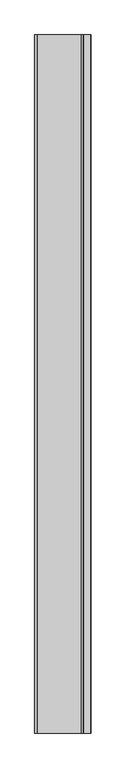
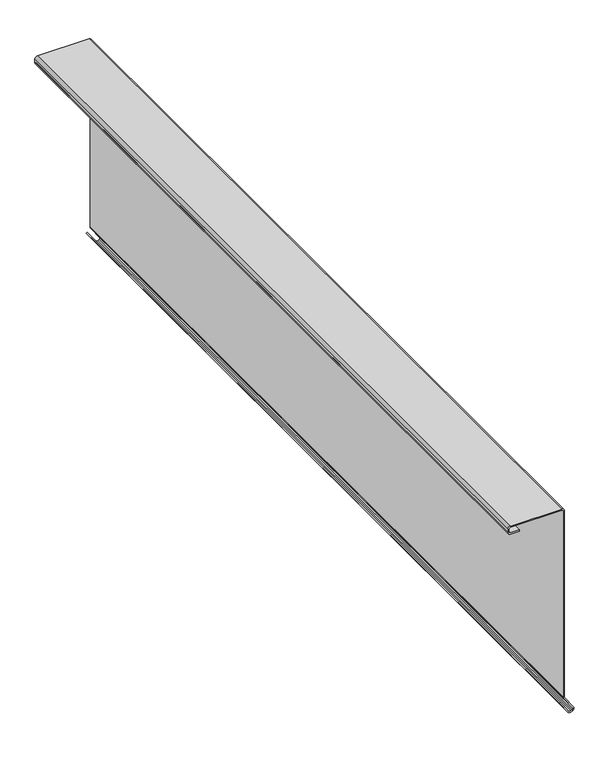
"""IFC4 building model written with IfcOpenShell, lengths in millimetres: proxy geometry, Flashing18:Flashing024:302126 : Flashing18:Flashing024:302126."""

from ifc_helpers import new_model, si_unit, point, frame, frame_2d, origin, place, context, project, spatial, polyline, circle_curve, trimmed, segment, composite_curve, outline, extrude, source, transform, mapped, element, save


def generic_models_c848868d(model_context):
    return source(origin(), model_context, "Body", "SweptSolid", [
        extrude(outline(composite_curve([segment(polyline([(41350.6549147, 10934.2276149), (41320.2092308, 10955.7821514)]), True, "CONTINUOUS"), segment(trimmed(circle_curve(frame_2d((41323.8783762, 10960.9648024)), 6.35), [point((41320.2092308, 10955.7821514))], [point((41318.4012804, 10964.1778884))], False, "CARTESIAN"), True, "CONTINUOUS"), segment(polyline([(41318.4012804, 10964.1778884), (41320.1425067, 10967.1460205)]), True, "CONTINUOUS"), segment(trimmed(circle_curve(frame_2d((41325.6196026, 10963.9329345)), 6.35), [point((41320.1425067, 10967.1460205))], [point((41329.2370767, 10969.1517831))], False, "CARTESIAN"), True, "CONTINUOUS"), segment(polyline([(41329.2370767, 10969.1517831), (41359.2301171, 10948.3619391)]), True, "CONTINUOUS"), segment(trimmed(circle_curve(frame_2d((41362.8475913, 10953.5807877)), 6.35), [point((41359.2301171, 10948.3619391))], [point((41362.8475913, 10947.2307877))], True, "CARTESIAN"), True, "CONTINUOUS"), segment(polyline([(41362.8475913, 10947.2307877), (41842.9189039, 10947.2307877)]), True, "CONTINUOUS"), segment(trimmed(circle_curve(frame_2d((41842.9189039, 10940.8807877)), 6.35), [point((41842.9189039, 10947.2307877))], [point((41849.2689039, 10940.8807877))], False, "CARTESIAN"), True, "CONTINUOUS"), segment(polyline([(41849.2689039, 10940.8807877), (41849.2689039, 10815.1631684)]), True, "CONTINUOUS"), segment(trimmed(circle_curve(frame_2d((41842.9189039, 10815.1631684)), 6.35), [point((41849.2689039, 10815.1631684))], [point((41842.9189039, 10808.8131684))], False, "CARTESIAN"), True, "CONTINUOUS"), segment(polyline([(41842.9189039, 10808.8131684), (41835.0524976, 10808.8131684)]), True, "CONTINUOUS"), segment(trimmed(circle_curve(frame_2d((41835.0524976, 10815.1631684)), 6.35), [point((41835.0524976, 10808.8131684))], [point((41828.7024976, 10815.1631684))], False, "CARTESIAN"), True, "CONTINUOUS"), segment(polyline([(41828.7024976, 10815.1631684), (41828.7024976, 10837.1896333), (41831.7024976, 10837.1896333), (41831.7024976, 10815.1631685)]), True, "CONTINUOUS"), segment(trimmed(circle_curve(frame_2d((41835.0524976, 10815.1631685)), 3.35), [point((41831.7024976, 10815.1631685))], [point((41835.0524976, 10811.8131685))], True, "CARTESIAN"), True, "CONTINUOUS"), segment(polyline([(41835.0524976, 10811.8131685), (41842.9189039, 10811.8131685)]), True, "CONTINUOUS"), segment(trimmed(circle_curve(frame_2d((41842.9189039, 10815.1631685)), 3.35), [point((41842.9189039, 10811.8131685))], [point((41846.2689039, 10815.1631685))], True, "CARTESIAN"), True, "CONTINUOUS"), segment(polyline([(41846.2689039, 10815.1631685), (41846.2689039, 10940.8807877)]), True, "CONTINUOUS"), segment(trimmed(circle_curve(frame_2d((41842.9189039, 10940.8807877)), 3.35), [point((41846.2689039, 10940.8807877))], [point((41842.9189039, 10944.2307877))], True, "CARTESIAN"), True, "CONTINUOUS"), segment(polyline([(41842.9189039, 10944.2307877), (41362.8475913, 10944.2307877)]), True, "CONTINUOUS"), segment(trimmed(circle_curve(frame_2d((41362.8475913, 10953.5807877)), 9.35), [point((41362.8475913, 10944.2307877))], [point((41357.5210742, 10945.8963413))], False, "CARTESIAN"), True, "CONTINUOUS"), segment(polyline([(41357.5210742, 10945.8963413), (41327.5280338, 10966.6861854)]), True, "CONTINUOUS"), segment(trimmed(circle_curve(frame_2d((41325.6196026, 10963.9329345)), 3.35), [point((41327.5280338, 10966.6861854))], [point((41322.730111, 10965.6280271))], True, "CARTESIAN"), True, "CONTINUOUS"), segment(polyline([(41322.730111, 10965.6280271), (41320.9888847, 10962.659895)]), True, "CONTINUOUS"), segment(trimmed(circle_curve(frame_2d((41323.8783762, 10960.9648024)), 3.35), [point((41320.9888847, 10962.659895))], [point((41321.9426853, 10958.2306479))], True, "CARTESIAN"), True, "CONTINUOUS"), segment(polyline([(41321.9426853, 10958.2306479), (41352.3883692, 10936.6761115), (41350.6549147, 10934.2276149)]), True, "CONTINUOUS")], self_intersect=False)), frame((0.0, 2495.6935399, 0.0), z_axis=(0.0, 1.0, 0.0), x_axis=(0.0, 0.0, 1.0)), (0.0, 0.0, 1.0), 2000.0),
    ])


if __name__ == "__main__":
    model = new_model("IFC4")
    model_context = context("Model", 3, world=origin())
    ifc_project = project(units=[si_unit("LENGTHUNIT", "METRE", prefix="MILLI")], contexts=[model_context])
    site = spatial("IfcSite", under=ifc_project)
    building = spatial("IfcBuilding", under=site)
    placement = place(None, origin())
    generic_models_shape = generic_models_c848868d(model_context)
    element("IfcBuildingElementProxy", 1, Name="Flashing18:Flashing024:302126 : Flashing18:Flashing024:302126", ObjectType="Flashing18:Flashing024:302126 : Flashing18:Flashing024:302126", at=placement, inside=building, context=model_context, shape_type="MappedRepresentation", body=[
        mapped(generic_models_shape, transform((0.0, 0.0, 0.0), x_axis=(1.0, 0.0, 0.0), y_axis=(0.0, 1.0, 0.0), z_axis=(0.0, 0.0, 1.0))),
    ])
    save(model, "model.ifc")

# Revit data of these elements
# Type "Flashing18:Flashing024:302126 : Flashing18:Flashing024:302126"
#   NameOverride = "Flashing18:Flashing024:302126"
#   ObjectTypeOverride = "Flashing18:Flashing024"
#   Reference = "Flashing024"
#   Category = "Generic Models"
#   Tag = "302126"
# Element 1 (IfcBuildingElementProxy, "Flashing18:Flashing024:302126 : Flashing18:Flashing024:302126")
#   Materials on its faces: "BRAKE METAL EAVE TRIM TO MATCH STANDING SEAM COLOR"
# Materials
#   "BRAKE METAL EAVE TRIM TO MATCH STANDING SEAM COLOR": class "Unassigned", colour RGB 128 128 128, transparency 0, Cost = 0
